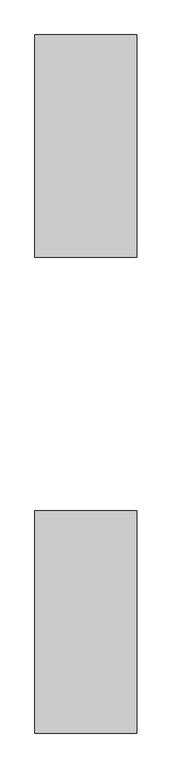
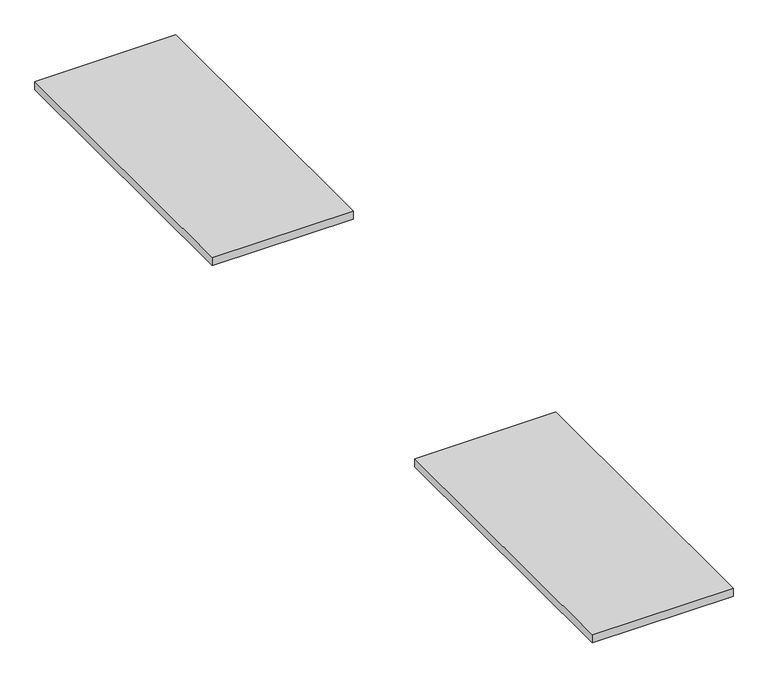
"""IFC4 building model written with IfcOpenShell, lengths in millimetres: furniture geometry, Desktop : Desktop."""

from ifc_helpers import new_model, si_unit, frame, origin, place, context, project, spatial, polyline, outline, extrude, source, transform, mapped, element, save


def furniture_681b888c(model_context):
    return source(origin(), model_context, "Body", "SweptSolid", [
        extrude(outline(polyline([(-7451.7086735, -5883.9860107), (-8074.0086735, -5883.9860107), (-8074.0086735, -4526.5757069), (-7451.7086735, -4526.5757069), (-7451.7086735, -5883.9860107)])), frame((0.0, 0.0, 723.9), z_axis=(0.0, 0.0, 1.0), x_axis=(1.0, 0.0, 0.0)), (0.0, 0.0, 1.0), 38.1),
        extrude(outline(polyline([(-7451.7086735, -2975.6860107), (-8074.0086735, -2975.6860107), (-8074.0086735, -1618.2757069), (-7451.7086735, -1618.2757069), (-7451.7086735, -2975.6860107)])), frame((0.0, 0.0, 723.9), z_axis=(0.0, 0.0, 1.0), x_axis=(1.0, 0.0, 0.0)), (0.0, 0.0, 1.0), 38.1),
    ])


if __name__ == "__main__":
    model = new_model("IFC4")
    model_context = context("Model", 3, world=origin())
    ifc_project = project(units=[si_unit("LENGTHUNIT", "METRE", prefix="MILLI")], contexts=[model_context])
    site = spatial("IfcSite", under=ifc_project)
    building = spatial("IfcBuilding", under=site)
    placement = place(None, origin())
    furniture_shape = furniture_681b888c(model_context)
    element("IfcFurniture", 1, ObjectType="Desktop : Desktop", at=placement, inside=building, context=model_context, shape_type="MappedRepresentation", body=[
        mapped(furniture_shape, transform((0.0, 0.0, 0.0), x_axis=(1.0, 0.0, 0.0), y_axis=(0.0, 1.0, 0.0), z_axis=(0.0, 0.0, 1.0))),
    ])
    save(model, "model.ifc")
